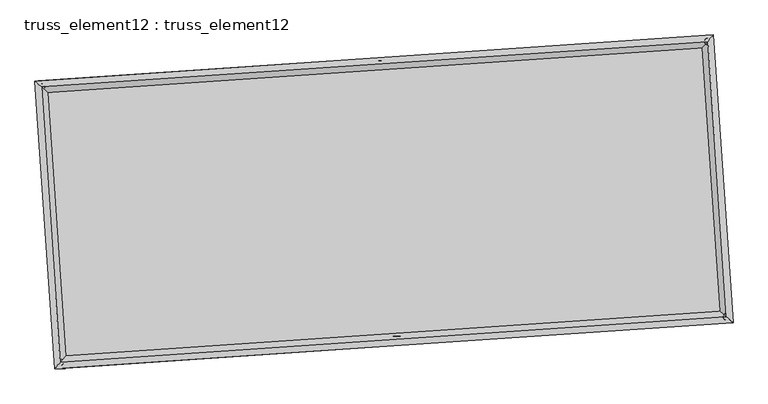
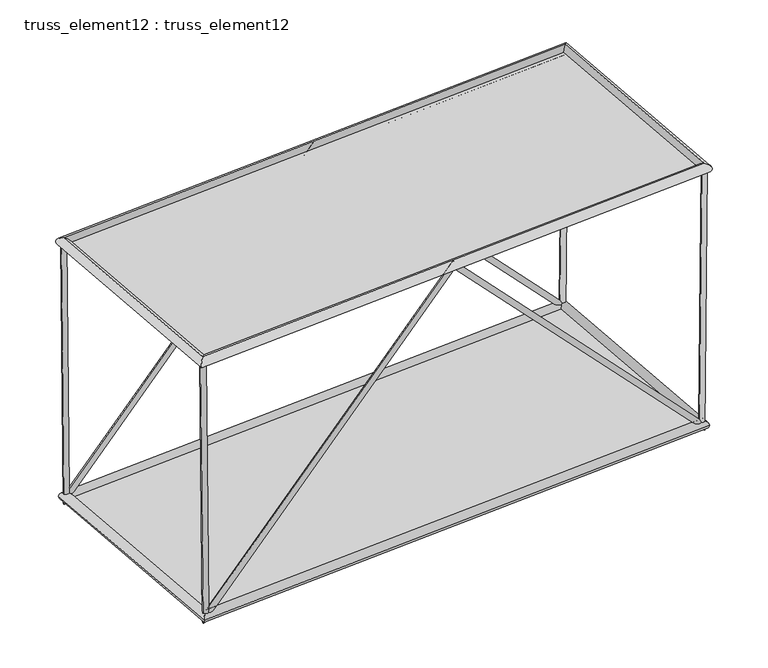
"""IFC4 building model written with IfcOpenShell, lengths in millimetres: plate geometry, truss_element12 : truss_element12."""

from ifc_helpers import new_model, si_unit, frame, origin, origin_with_axes, place, context, project, spatial, polyline, circle_curve, ellipse_curve, outline, extrude, source, transform, mapped, element, save
from ifc_brep_helpers import plane_surface, cylinder_surface, advanced_brep


def truss_element12_truss_element12_ac9c6d62(model_context):
    return source(origin(), model_context, "Body", "SolidModel", [
        advanced_brep(
        [(-3716.0930721, 2272.7361645, 5000.2487185), (-3815.1912006, 2259.3752454, 4999.2255971), (-3666.1964298, 2276.1384269, 122.8985351), (-3762.790453, 2262.9482532, -122.8985351), (1063.2705222, 2598.6227999, 5071.8637093), (1063.7254289, 2592.0500239, 4927.6196851), (5793.6135203, 2921.1669073, 122.9048123), (5891.1474567, 2921.2135812, -122.9048123), (5842.6407291, 2924.5098863, 5000.248885), (5942.6354458, 2924.7243515, 4999.2435881)],
        [
            (0, 1, circle_curve(frame((-3765.6421364, 2266.055705, 4999.7371578), z_axis=(-0.010229738989149566, -0.0006975270147916147, 0.9999474315664186), x_axis=(-0.13360930371043286, 0.991033852899563, -0.0006755509311635323)), 50.0)),
            (1, 0, circle_curve(frame((-3765.6421364, 2266.055705, 4999.7371578), z_axis=(-0.010229738989149566, -0.0006975270147916147, 0.9999474315664186), x_axis=(-0.13360930371043286, 0.991033852899563, -0.0006755509311635323)), 50.0)),
            (0, 2),
            (2, 3, ellipse_curve(frame((-3714.4934414, 2269.54334, 0.0), z_axis=(-0.9276876380424472, -0.06325549356725499, 0.36795976513307577), x_axis=(0.367107348096881, 0.02503165456104934, 0.9298417130045371)), 132.4592623, 50.0)),
            (3, 1),
            (3, 2, ellipse_curve(frame((-3714.4934414, 2269.54334, 0.0), z_axis=(-0.9276876380424472, -0.06325549356725499, 0.36795976513307577), x_axis=(0.367107348096881, 0.02503165456104934, 0.9298417130045371)), 132.4592623, 50.0)),
            (2, 4),
            (4, 5, ellipse_curve(frame((1063.4979755, 2595.3364119, 4999.7416972), z_axis=(-0.9976833949926481, -0.0680282381549069, -4.657770887694116e-05), x_axis=(4.6469806773723855e-05, 3.1685994757026087e-06, -0.9999999989152586)), 72.2790583, 50.0)),
            (5, 3),
            (5, 4, ellipse_curve(frame((1063.4979755, 2595.3364119, 4999.7416972), z_axis=(-0.9976833949926481, -0.0680282381549069, -4.657770887694116e-05), x_axis=(4.6469806773723855e-05, 3.1685994757026087e-06, -0.9999999989152586)), 72.2790583, 50.0)),
            (4, 6),
            (6, 7, ellipse_curve(frame((5842.3804885, 2921.1902443, 0.0), z_axis=(-0.9276377400160161, -0.06325209121051292, -0.3680861261382656), x_axis=(-0.3672334163736703, -0.025040250677613285, 0.9297916991157348)), 132.4731533, 50.0)),
            (7, 5),
            (7, 6, ellipse_curve(frame((5842.3804885, 2921.1902443, 0.0), z_axis=(-0.9276377400160161, -0.06325209121051292, -0.3680861261382656), x_axis=(-0.3672334163736703, -0.025040250677613285, 0.9297916991157348)), 132.4731533, 50.0)),
            (8, 9, circle_curve(frame((5892.6380875, 2924.6171189, 4999.7462366), z_axis=(0.010051519791738127, 0.000685374925194703, 0.9999492473176268), x_axis=(-0.0021514333546637375, 0.9999974653609742, -0.0006637817017735374)), 50.0)),
            (9, 8, circle_curve(frame((5892.6380875, 2924.6171189, 4999.7462366), z_axis=(0.010051519791738127, 0.000685374925194703, 0.9999492473176268), x_axis=(-0.0021514333546637375, 0.9999974653609742, -0.0006637817017735374)), 50.0)),
            (6, 8),
            (9, 7),
        ],
        [
            plane_surface(frame((-3765.6421364, 2316.0556928, 4999.772036), z_axis=(-0.01022973898914786, -0.0006975270147901555, 0.9999474315664189), x_axis=(0.9999476748511464, -7.13589268563908e-06, 0.010229736500278365))),
            cylinder_surface(frame((-3765.6421364, 2266.055705, 4999.7371578), z_axis=(-0.010229738989149566, -0.0006975270147916147, 0.9999474315664186), x_axis=(-0.13360930371043286, 0.991033852899563, -0.0006755509311635323)), 50.0),
            cylinder_surface(frame((-3714.4934414, 2269.54334, 0.0), z_axis=(-0.6901272026448979, -0.047057150529254535, -0.722156540338447), x_axis=(-0.02041139550442059, 0.9987523879545969, -0.04557458160589792)), 50.0),
            cylinder_surface(frame((1063.4979755, 2595.3364119, 4999.7416972), z_axis=(-0.6901943166001666, -0.047061726774740395, 0.7220920988390669), x_axis=(-0.11534522502427148, 0.9922792109969094, -0.04557901367352192)), 50.0),
            plane_surface(frame((5892.6380875, 2874.6171306, 4999.7805071), z_axis=(0.010051519791740156, 0.0006853749251952957, 0.9999492473176268), x_axis=(0.9999494821989141, -6.889407663024368e-06, -0.010051517430706975))),
            cylinder_surface(frame((5842.3804885, 2921.1902443, 0.0), z_axis=(-0.010051519791738127, -0.000685374925194703, -0.9999492473176268), x_axis=(-0.0021514333546637375, 0.9999974653609742, -0.0006637817017735374)), 50.0),
        ],
        [
            (0, [[1, 2]]),
            (1, [[-1, 3, 4, 5]]),
            (1, [[-2, -5, 6, -3]]),
            (2, [[-4, 7, 8, 9]]),
            (2, [[-6, -9, 10, -7]]),
            (3, [[-8, 11, 12, 13]]),
            (3, [[-10, -13, 14, -11]]),
            (4, [[15, 16]]),
            (5, [[-12, 17, -16, 18]]),
            (5, [[-14, -18, -15, -17]]),
        ],
    ),
        advanced_brep(
        [(-3443.9801192, -1717.9974198, 5000.2487185), (-3543.0782477, -1731.3583389, 4999.2255971), (-3394.0834769, -1714.5951574, 122.8985351), (-3490.6775001, -1727.7853311, -122.8985351), (1335.3834751, -1392.1107844, 5071.8637093), (1335.8383818, -1398.6835604, 4927.6196851), (6065.7264732, -1069.566677, 122.9048123), (6163.2604096, -1069.5200031, -122.9048123), (6114.753682, -1066.223698, 5000.248885), (6214.7483988, -1066.0092328, 4999.2435881)],
        [
            (0, 1, circle_curve(frame((-3493.5291834, -1724.6778793, 4999.7371578), z_axis=(-0.010229738989149568, -0.0006975270147916012, 0.9999474315664186), x_axis=(-0.1336093037104329, 0.991033852899563, -0.0006755509311635461)), 50.0)),
            (1, 0, circle_curve(frame((-3493.5291834, -1724.6778793, 4999.7371578), z_axis=(-0.010229738989149568, -0.0006975270147916012, 0.9999474315664186), x_axis=(-0.1336093037104329, 0.991033852899563, -0.0006755509311635461)), 50.0)),
            (0, 2),
            (2, 3, ellipse_curve(frame((-3442.3804885, -1721.1902443, 0.0), z_axis=(-0.9276876380424474, -0.06325549356725498, 0.3679597651330757), x_axis=(0.3671073480968811, 0.025031654561049346, 0.9298417130045371)), 132.4592623, 50.0)),
            (3, 1),
            (3, 2, ellipse_curve(frame((-3442.3804885, -1721.1902443, 0.0), z_axis=(-0.9276876380424474, -0.06325549356725498, 0.3679597651330757), x_axis=(0.3671073480968811, 0.025031654561049346, 0.9298417130045371)), 132.4592623, 50.0)),
            (2, 4),
            (4, 5, ellipse_curve(frame((1335.6109285, -1395.3971724, 4999.7416972), z_axis=(-0.9976833949926481, -0.06802823815490679, -4.657770887694117e-05), x_axis=(4.6469806773723855e-05, 3.1685994756065187e-06, -0.9999999989152586)), 72.2790583, 50.0)),
            (5, 3),
            (5, 4, ellipse_curve(frame((1335.6109285, -1395.3971724, 4999.7416972), z_axis=(-0.9976833949926481, -0.06802823815490679, -4.657770887694117e-05), x_axis=(4.6469806773723855e-05, 3.1685994756065187e-06, -0.9999999989152586)), 72.2790583, 50.0)),
            (4, 6),
            (6, 7, ellipse_curve(frame((6114.4934414, -1069.54334, 0.0), z_axis=(-0.9276377400160161, -0.0632520912105128, -0.3680861261382654), x_axis=(-0.3672334163736703, -0.02504025067761318, 0.9297916991157348)), 132.4731533, 50.0)),
            (7, 5),
            (7, 6, ellipse_curve(frame((6114.4934414, -1069.54334, 0.0), z_axis=(-0.9276377400160161, -0.0632520912105128, -0.3680861261382654), x_axis=(-0.3672334163736703, -0.02504025067761318, 0.9297916991157348)), 132.4731533, 50.0)),
            (8, 9, circle_curve(frame((6164.7510404, -1066.1164654, 4999.7462366), z_axis=(0.010051519791738519, 0.0006853749251947742, 0.9999492473176269), x_axis=(-0.0021514333546638212, 0.9999974653609742, -0.0006637817017736069)), 50.0)),
            (9, 8, circle_curve(frame((6164.7510404, -1066.1164654, 4999.7462366), z_axis=(0.010051519791738519, 0.0006853749251947742, 0.9999492473176269), x_axis=(-0.0021514333546638212, 0.9999974653609742, -0.0006637817017736069)), 50.0)),
            (6, 8),
            (9, 7),
        ],
        [
            plane_surface(frame((-3493.5291834, -1674.6778915, 4999.772036), z_axis=(-0.01022973898914786, -0.0006975270147901575, 0.9999474315664189), x_axis=(0.9999476748511464, -7.13589268563908e-06, 0.010229736500278365))),
            cylinder_surface(frame((-3493.5291834, -1724.6778793, 4999.7371578), z_axis=(-0.010229738989149568, -0.0006975270147916012, 0.9999474315664186), x_axis=(-0.1336093037104329, 0.991033852899563, -0.0006755509311635461)), 50.0),
            cylinder_surface(frame((-3442.3804885, -1721.1902443, 0.0), z_axis=(-0.6901272026448979, -0.04705715052925453, -0.7221565403384471), x_axis=(-0.02041139550442058, 0.9987523879545969, -0.04557458160589791)), 50.0),
            cylinder_surface(frame((1335.6109285, -1395.3971724, 4999.7416972), z_axis=(-0.6901943166001666, -0.047061726774740256, 0.7220920988390671), x_axis=(-0.11534522502427137, 0.9922792109969095, -0.04557901367352197)), 50.0),
            plane_surface(frame((6164.7510404, -1116.1164537, 4999.7805071), z_axis=(0.010051519791740156, 0.0006853749251952975, 0.9999492473176268), x_axis=(0.9999494821989141, -6.889407663024368e-06, -0.010051517430706975))),
            cylinder_surface(frame((6114.4934414, -1069.54334, 0.0), z_axis=(-0.010051519791738517, -0.0006853749251947741, -0.9999492473176267), x_axis=(-0.0021514333546638212, 0.9999974653609742, -0.0006637817017736069)), 50.0),
        ],
        [
            (0, [[1, 2]]),
            (1, [[-1, 3, 4, 5]]),
            (1, [[-2, -5, 6, -3]]),
            (2, [[-4, 7, 8, 9]]),
            (2, [[-6, -9, 10, -7]]),
            (3, [[-8, 11, 12, 13]]),
            (3, [[-10, -13, 14, -11]]),
            (4, [[15, 16]]),
            (5, [[-12, 17, -16, 18]]),
            (5, [[-14, -18, -15, -17]]),
        ],
    ),
        advanced_brep(
        [(-3493.526795, -1724.6752322, 4909.7371579), (-3493.5315719, -1724.6805265, 5089.7371578), (-3765.644862, 2266.0580034, 5089.7371578), (-3765.6394107, 2266.0534065, 4909.7371579), (5892.6403075, 2924.6197546, 5089.7462366), (5892.6358675, 2924.6144832, 4909.7462366), (6164.7535976, -1066.1187754, 5089.7462366), (6164.7484832, -1066.1141555, 4909.7462366)],
        [
            (0, 1, ellipse_curve(frame((-3493.5291834, -1724.6778793, 4999.7371578), z_axis=(-0.7535719234051438, 0.6573654662781065, -6.631385733945912e-07), x_axis=(-0.6573654662777754, -0.7535719234054328, -6.631385733946736e-07)), 127.2792206, 90.0)),
            (1, 2),
            (2, 3, ellipse_curve(frame((-3765.6421364, 2266.055705, 4999.7371578), z_axis=(-0.6573654662777749, -0.753571923405433, -6.631385733947504e-07), x_axis=(0.753571923405144, -0.6573654662781062, 6.631385733946685e-07)), 127.2792206, 90.0)),
            (3, 0),
            (1, 0, ellipse_curve(frame((-3493.5291834, -1724.6778793, 4999.7371578), z_axis=(-0.7535719234051438, 0.6573654662781065, -6.631385733945912e-07), x_axis=(-0.6573654662777754, -0.7535719234054328, -6.631385733946736e-07)), 127.2792206, 90.0)),
            (3, 2, ellipse_curve(frame((-3765.6421364, 2266.055705, 4999.7371578), z_axis=(-0.6573654662777749, -0.753571923405433, -6.631385733947504e-07), x_axis=(0.753571923405144, -0.6573654662781062, 6.631385733946685e-07)), 127.2792206, 90.0)),
            (2, 4),
            (4, 5, ellipse_curve(frame((5892.6380875, 2924.6171189, 4999.7462366), z_axis=(-0.7535719234051438, 0.6573654662781065, -6.631385733947457e-07), x_axis=(-0.657365466277775, -0.7535719234054329, -6.63138573394673e-07)), 127.2792206, 90.0)),
            (5, 3),
            (5, 4, ellipse_curve(frame((5892.6380875, 2924.6171189, 4999.7462366), z_axis=(-0.7535719234051438, 0.6573654662781065, -6.631385733947457e-07), x_axis=(-0.657365466277775, -0.7535719234054329, -6.63138573394673e-07)), 127.2792206, 90.0)),
            (4, 6),
            (6, 7, ellipse_curve(frame((6164.7510404, -1066.1164654, 4999.7462366), z_axis=(0.6573654662777753, 0.7535719234054328, 6.631385733945962e-07), x_axis=(-0.7535719234051438, 0.6573654662781064, -6.631385733946685e-07)), 127.2792206, 90.0)),
            (7, 5),
            (7, 6, ellipse_curve(frame((6164.7510404, -1066.1164654, 4999.7462366), z_axis=(0.6573654662777753, 0.7535719234054328, 6.631385733945962e-07), x_axis=(-0.7535719234051438, 0.6573654662781064, -6.631385733946685e-07)), 127.2792206, 90.0)),
            (6, 1),
            (0, 7),
        ],
        [
            cylinder_surface(frame((-3493.5291834, -1724.6778793, 4999.7371578), z_axis=(0.06802823822869494, -0.997683396074877, 0.0), x_axis=(-0.9976833956703363, -0.06802823820111085, -2.8477362265498946e-05)), 90.0),
            cylinder_surface(frame((-3765.6421364, 2266.055705, 4999.7371578), z_axis=(-0.9976833960744383, -0.06802823822866604, -9.378195642275444e-07), x_axis=(-0.06802823817713145, 0.9976833956982993, -2.7539542701627088e-05)), 90.0),
            cylinder_surface(frame((5892.6380875, 2924.6171189, 4999.7462366), z_axis=(-0.06802823822869457, 0.9976833960748772, 0.0), x_axis=(0.997683395721871, 0.06802823820462442, -2.6601723137755227e-05)), 90.0),
            cylinder_surface(frame((6164.7510404, -1066.1164654, 4999.7462366), z_axis=(0.9976833960744383, 0.06802823822866567, 9.378195642274352e-07), x_axis=(0.06802823822866567, -0.9976833956947854, -2.753954270162708e-05)), 90.0),
        ],
        [
            (0, [[1, 2, 3, 4]]),
            (0, [[5, -4, 6, -2]]),
            (1, [[-3, 7, 8, 9]]),
            (1, [[-6, -9, 10, -7]]),
            (2, [[-8, 11, 12, 13]]),
            (2, [[-10, -13, 14, -11]]),
            (3, [[-12, 15, -1, 16]]),
            (3, [[-14, -16, -5, -15]]),
        ],
    ),
        advanced_brep(
        [(-3358.7115243, -1625.2761972, 0.0), (-3526.0494527, -1817.1042913, 0.0), (-3810.4074885, 2353.2123043, 0.0), (-3618.5793943, 2185.8743758, 0.0), (5926.0494527, 3017.1042913, 0.0), (5758.7115243, 2825.2761972, 0.0), (6210.4074885, -1153.2123043, 0.0), (6018.5793943, -985.8743758, 0.0)],
        [
            (0, 1, ellipse_curve(frame((-3442.3804885, -1721.1902443, 0.0), z_axis=(-0.7535719234054566, 0.6573654662780822, 0.0), x_axis=(-0.6573654662780821, -0.7535719234054568, 0.0)), 127.2792206, 90.0)),
            (1, 2),
            (2, 3, ellipse_curve(frame((-3714.4934414, 2269.54334, 0.0), z_axis=(-0.6573654662780822, -0.7535719234054568, 0.0), x_axis=(0.7535719234054568, -0.6573654662780821, 0.0)), 127.2792206, 90.0)),
            (3, 0),
            (1, 0, ellipse_curve(frame((-3442.3804885, -1721.1902443, 0.0), z_axis=(-0.7535719234054566, 0.6573654662780822, 0.0), x_axis=(-0.6573654662780821, -0.7535719234054568, 0.0)), 127.2792206, 90.0)),
            (3, 2, ellipse_curve(frame((-3714.4934414, 2269.54334, 0.0), z_axis=(-0.6573654662780822, -0.7535719234054568, 0.0), x_axis=(0.7535719234054568, -0.6573654662780821, 0.0)), 127.2792206, 90.0)),
            (2, 4),
            (4, 5, ellipse_curve(frame((5842.3804885, 2921.1902443, 0.0), z_axis=(-0.7535719234054566, 0.6573654662780823, 0.0), x_axis=(-0.6573654662780822, -0.7535719234054566, 0.0)), 127.2792206, 90.0)),
            (5, 3),
            (5, 4, ellipse_curve(frame((5842.3804885, 2921.1902443, 0.0), z_axis=(-0.7535719234054566, 0.6573654662780823, 0.0), x_axis=(-0.6573654662780822, -0.7535719234054566, 0.0)), 127.2792206, 90.0)),
            (4, 6),
            (6, 7, ellipse_curve(frame((6114.4934414, -1069.54334, 0.0), z_axis=(0.6573654662780825, 0.7535719234054565, 0.0), x_axis=(-0.7535719234054565, 0.6573654662780825, 0.0)), 127.2792206, 90.0)),
            (7, 5),
            (7, 6, ellipse_curve(frame((6114.4934414, -1069.54334, 0.0), z_axis=(0.6573654662780825, 0.7535719234054565, 0.0), x_axis=(-0.7535719234054565, 0.6573654662780825, 0.0)), 127.2792206, 90.0)),
            (6, 1),
            (0, 7),
        ],
        [
            cylinder_surface(frame((-3442.3804885, -1721.1902443, 0.0), z_axis=(0.06802823822869897, -0.9976833960748768, 0.0), x_axis=(-0.9976833960748768, -0.06802823822869897, 0.0)), 90.0),
            cylinder_surface(frame((-3714.4934414, 2269.54334, 0.0), z_axis=(-0.9976833960748768, -0.06802823822869992, 0.0), x_axis=(-0.06802823822869992, 0.9976833960748768, 0.0)), 90.0),
            cylinder_surface(frame((5842.3804885, 2921.1902443, 0.0), z_axis=(-0.06802823822869855, 0.9976833960748768, 0.0), x_axis=(0.9976833960748768, 0.06802823822869855, 0.0)), 90.0),
            cylinder_surface(frame((6114.4934414, -1069.54334, 0.0), z_axis=(0.9976833960748768, 0.06802823822869959, 0.0), x_axis=(0.06802823822869959, -0.9976833960748768, 0.0)), 90.0),
        ],
        [
            (0, [[1, 2, 3, 4]]),
            (0, [[5, -4, 6, -2]]),
            (1, [[-3, 7, 8, 9]]),
            (1, [[-6, -9, 10, -7]]),
            (2, [[-8, 11, 12, 13]]),
            (2, [[-10, -13, 14, -11]]),
            (3, [[-12, 15, -1, 16]]),
            (3, [[-14, -16, -5, -15]]),
        ],
    ),
        extrude(outline(polyline([(-3442.3804885, -1721.1902443), (-3714.4934414, 2269.54334), (5842.3804885, 2921.1902443), (6114.4934414, -1069.54334), (-3442.3804885, -1721.1902443)])), origin_with_axes(), (0.0, 0.0, 1.0), 20.0),
        extrude(outline(polyline([(-2000.0, 4840.3532933), (2000.0, 4840.3532934), (2000.0, -4840.3532934), (-2000.0, -4840.3532934), (-2000.0, 4840.3532933)])), frame((1199.554452, 599.9696198, 4999.7416972), z_axis=(-9.356470077439426e-07, -6.379821273080194e-08, 0.9999999999995604), x_axis=(-0.06802823822869858, 0.9976833960748768, 0.0)), (0.0, 0.0, 1.0), 20.0),
    ])


if __name__ == "__main__":
    model = new_model("IFC4")
    model_context = context("Model", 3, world=origin())
    ifc_project = project(units=[si_unit("LENGTHUNIT", "METRE", prefix="MILLI")], contexts=[model_context])
    site = spatial("IfcSite", under=ifc_project)
    building = spatial("IfcBuilding", under=site)
    placement = place(None, origin())
    truss_element12_truss_element12_shape = truss_element12_truss_element12_ac9c6d62(model_context)
    element("IfcPlate", 1, ObjectType="truss_element12 : truss_element12", at=placement, inside=building, context=model_context, shape_type="MappedRepresentation", body=[
        mapped(truss_element12_truss_element12_shape, transform((0.0, 0.0, 0.0), x_axis=(1.0, 0.0, 0.0), y_axis=(0.0, 1.0, 0.0), z_axis=(0.0, 0.0, 1.0))),
    ])
    save(model, "model.ifc")

# Revit data of these elements
# Type "truss_element12 : truss_element12"
#   steellbar1 = 90 mm
#   steelbar2 = 50 mm
#   offset1 = 5000 mm
#   M = Default Roof
# Element 1 (IfcPlate, "truss_element12 : truss_element12")
#   Materials on its faces: "Default Roof"
# Materials
#   "Default Roof": class "Miscellaneous", colour RGB 0 127 0, transparency 0, Comments = "Rendering appearance not upgraded Rendering appearance not upgraded ", Cost = 0
